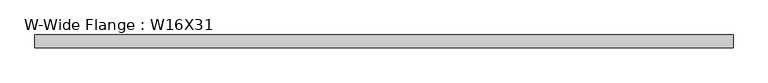
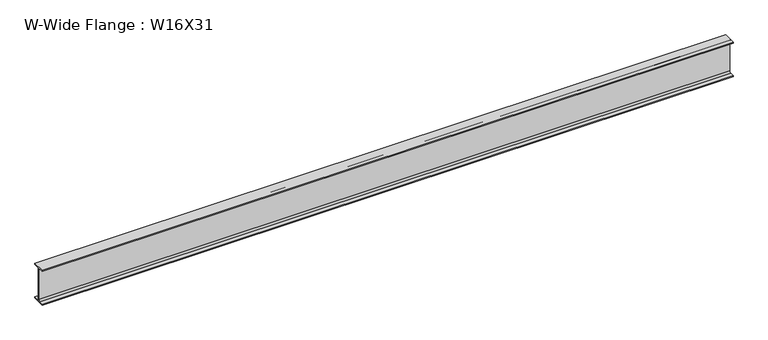
"""IFC4 building model written with IfcOpenShell, lengths in millimetres: beam geometry, W-Wide Flange : W16X31."""

import ifcopenshell
import ifcopenshell.guid

model = None  # the IFC model being written
_history = None  # IfcOwnerHistory: only IFC2X3 demands one
_inside = {}  # id of a spatial element -> (the spatial element, [elements in it])
_under = {}  # id of a project, library or spatial element -> (it, [spatial elements below it])
_declared = {}  # id of a project -> (the project, [libraries it declares])
_typed = {}  # id of a type object -> (the type object, [elements of that type])
_made_of = {}  # id of a material, layer set ... -> (it, [elements and type objects made of it])


def new_model(schema):
    """Start an empty IFC model of exactly this schema.

    Asked for "IFC4X3", IfcOpenShell would pick the latest addendum, in which some entities
    have other attributes; the version numbers below select the first issue.
    IFC2X3 requires an IfcOwnerHistory on every rooted entity: one is made here for all.
    """
    global model, _history
    if schema == "IFC4X3":
        model = ifcopenshell.file(schema_version=(4, 3, 0, 0))
    else:
        model = ifcopenshell.file(schema=schema)
    _inside.clear()
    _under.clear()
    _declared.clear()
    _typed.clear()
    _made_of.clear()
    _history = None
    if model.schema == "IFC2X3":
        org = make("IfcOrganization", Name="unknown")
        user = make(
            "IfcPersonAndOrganization",
            ThePerson=make("IfcPerson", FamilyName="unknown"),
            TheOrganization=org,
        )
        app = make(
            "IfcApplication",
            ApplicationDeveloper=org,
            Version="unknown",
            ApplicationFullName="unknown",
            ApplicationIdentifier="unknown",
        )
        _history = make(
            "IfcOwnerHistory",
            OwningUser=user,
            OwningApplication=app,
            ChangeAction="ADDED",
            CreationDate=0,
        )
    return model


def make(cls, **values):
    """One entity of the class cls with the attributes given. An attribute that is None is left unset."""
    return model.create_entity(
        cls, **{name: value for name, value in values.items() if value is not None}
    )


def rooted(cls, **values):
    """An entity with a GlobalId (a new one), such as an element, a storey or a relation."""
    return make(cls, GlobalId=ifcopenshell.guid.new(), OwnerHistory=_history, **values)


def si_unit(unit_type, name, prefix=None):
    """IfcSIUnit, for example si_unit("LENGTHUNIT", "METRE", prefix="MILLI")."""
    return make("IfcSIUnit", UnitType=unit_type, Prefix=prefix, Name=name)


def assignment(units):
    """IfcUnitAssignment: the units of a project."""
    return None if units is None else make("IfcUnitAssignment", Units=units)


def point(xyz):
    """IfcCartesianPoint."""
    return None if xyz is None else make("IfcCartesianPoint", Coordinates=xyz)


def direction(xyz):
    """IfcDirection."""
    return None if xyz is None else make("IfcDirection", DirectionRatios=xyz)


def frame(location, z_axis=None, x_axis=None):
    """IfcAxis2Placement3D, a coordinate frame: its origin and axes. An axis left out is left unset."""
    return make(
        "IfcAxis2Placement3D",
        Location=point(location),
        Axis=direction(z_axis),
        RefDirection=direction(x_axis),
    )


def frame_2d(location, x_axis=None):
    """IfcAxis2Placement2D, a coordinate frame in the plane: its origin and x axis."""
    return make(
        "IfcAxis2Placement2D", Location=point(location), RefDirection=direction(x_axis)
    )


def origin():
    """The frame at (0, 0, 0) with its axes left unset."""
    return frame((0.0, 0.0, 0.0))


def place(relative_to, where):
    """IfcLocalPlacement: puts the frame where relative to a parent placement (None: the world)."""
    return make(
        "IfcLocalPlacement", PlacementRelTo=relative_to, RelativePlacement=where
    )


def context(
    kind, dimensions, precision=None, world=None, true_north=None, identifier=None
):
    """IfcGeometricRepresentationContext, for example the 3D "Model" context."""
    return make(
        "IfcGeometricRepresentationContext",
        ContextIdentifier=identifier,
        ContextType=kind,
        CoordinateSpaceDimension=dimensions,
        Precision=precision,
        WorldCoordinateSystem=world,
        TrueNorth=true_north,
    )


def project(units=None, contexts=None):
    """IfcProject with its units and contexts."""
    return rooted(
        "IfcProject",
        Name="project",
        RepresentationContexts=contexts,
        UnitsInContext=assignment(units),
    )


def spatial(cls, under=None, at=None, **own):
    """A site, building, storey or space (cls), placed at a placement, below another one or the project."""
    s = rooted(cls, ObjectPlacement=at, **own)
    if under is not None:
        _under.setdefault(under.id(), (under, []))[1].append(s)
    return s


def polyline(points):
    """IfcPolyline through the points."""
    return make("IfcPolyline", Points=[point(p) for p in points])


def circle_curve(where, radius):
    """IfcCircle in the frame where."""
    return make("IfcCircle", Position=where, Radius=radius)


def trimmed(basis, trim1, trim2, sense, master):
    """IfcTrimmedCurve: the piece of a basis curve between two trims."""
    return make(
        "IfcTrimmedCurve",
        BasisCurve=basis,
        Trim1=trim1,
        Trim2=trim2,
        SenseAgreement=sense,
        MasterRepresentation=master,
    )


def segment(curve, same_sense, transition):
    """IfcCompositeCurveSegment."""
    return make(
        "IfcCompositeCurveSegment",
        Transition=transition,
        SameSense=same_sense,
        ParentCurve=curve,
    )


def composite_curve(segments, self_intersect=None):
    """IfcCompositeCurve: segments joined end to end."""
    return make("IfcCompositeCurve", Segments=segments, SelfIntersect=self_intersect)


def outline(outer, holes=None, kind="AREA"):
    """IfcArbitraryClosedProfileDef: a profile drawn as a closed curve; with holes, ...WithVoids."""
    if holes is None:
        return make("IfcArbitraryClosedProfileDef", ProfileType=kind, OuterCurve=outer)
    return make(
        "IfcArbitraryProfileDefWithVoids",
        ProfileType=kind,
        OuterCurve=outer,
        InnerCurves=holes,
    )


def extrude(swept, where, along, depth):
    """IfcExtrudedAreaSolid: the profile swept, set in the frame where, extruded along a direction by depth."""
    return make(
        "IfcExtrudedAreaSolid",
        SweptArea=swept,
        Position=where,
        ExtrudedDirection=direction(along),
        Depth=depth,
    )


def shape(context_of_items, identifier, shape_type, items):
    """IfcShapeRepresentation: the items that make up one representation, for example the "Body"."""
    return make(
        "IfcShapeRepresentation",
        ContextOfItems=context_of_items,
        RepresentationIdentifier=identifier,
        RepresentationType=shape_type,
        Items=items,
    )


def source(mapping_origin, context_of_items, identifier, shape_type, items):
    """IfcRepresentationMap: a shape defined once, which mapped items show again and again."""
    return make(
        "IfcRepresentationMap",
        MappingOrigin=mapping_origin,
        MappedRepresentation=shape(context_of_items, identifier, shape_type, items),
    )


def transform(
    local_origin,
    x_axis=None,
    y_axis=None,
    z_axis=None,
    scale=None,
    scale2=None,
    scale3=None,
    uniform=True,
):
    """IfcCartesianTransformationOperator3D, or its non-uniform kind. x_axis, y_axis, z_axis: its Axis1, 2, 3."""
    if uniform:
        return make(
            "IfcCartesianTransformationOperator3D",
            Axis1=direction(x_axis),
            Axis2=direction(y_axis),
            LocalOrigin=point(local_origin),
            Scale=scale,
            Axis3=direction(z_axis),
        )
    return make(
        "IfcCartesianTransformationOperator3DnonUniform",
        Axis1=direction(x_axis),
        Axis2=direction(y_axis),
        LocalOrigin=point(local_origin),
        Scale=scale,
        Axis3=direction(z_axis),
        Scale2=scale2,
        Scale3=scale3,
    )


def mapped(mapping_source, mapping_target):
    """IfcMappedItem: shows the shape of a source again, moved by a transform."""
    return make(
        "IfcMappedItem", MappingSource=mapping_source, MappingTarget=mapping_target
    )


def made_of(thing, what):
    """Note that an element or type object is made of a material, layer set ...; save() writes the relation."""
    if what is not None:
        _made_of.setdefault(what.id(), (what, []))[1].append(thing)
    return thing


def element(
    cls,
    number,
    at=None,
    inside=None,
    cuts=None,
    type_object=None,
    material=None,
    context=None,
    identifier="Body",
    shape_type=None,
    held_by="IfcProductDefinitionShape",
    body=None,
    shapes=None,
    **own,
):
    """One element of the class cls, such as IfcWall. Its Tag is "e" and its number.

    at: its placement. inside: the storey or other place that contains it. cuts: it is an
    opening in that element (IfcRelVoidsElement). A single representation is given by context,
    identifier, shape_type and body (its items); several are given by shapes. held_by: the class
    of the entity that holds the representations. save() writes the other relations.
    """
    e = rooted(cls, Tag="e%d" % number, ObjectPlacement=at, **own)
    if body is not None:
        shapes = [shape(context, identifier, shape_type, body)]
    if shapes is not None:
        e.Representation = make(held_by, Representations=shapes)
    if inside is not None:
        _inside.setdefault(inside.id(), (inside, []))[1].append(e)
    if cuts is not None:
        rooted(
            "IfcRelVoidsElement", RelatingBuildingElement=cuts, RelatedOpeningElement=e
        )
    if type_object is not None:
        _typed.setdefault(type_object.id(), (type_object, []))[1].append(e)
    return made_of(e, material)


def aggregate(whole, parts):
    """IfcRelAggregates: a whole, such as a stair, and the parts it consists of."""
    return rooted("IfcRelAggregates", RelatingObject=whole, RelatedObjects=parts)


def save(model, path):
    """Write the relations noted so far, then the file.

    IfcRelAggregates (storeys below a building ...), IfcRelContainedInSpatialStructure (elements
    in a storey), IfcRelDefinesByType, IfcRelAssociatesMaterial and IfcRelDeclares: one each for
    every whole, place, type object, material and project.
    """
    for whole, parts in _under.values():
        aggregate(whole, parts)
    for where, things in _inside.values():
        rooted(
            "IfcRelContainedInSpatialStructure",
            RelatedElements=things,
            RelatingStructure=where,
        )
    for kind, things in _typed.values():
        rooted("IfcRelDefinesByType", RelatedObjects=things, RelatingType=kind)
    for what, things in _made_of.values():
        rooted("IfcRelAssociatesMaterial", RelatedObjects=things, RelatingMaterial=what)
    for by, libraries in _declared.values():
        rooted("IfcRelDeclares", RelatingContext=by, RelatedDefinitions=libraries)
    model.write(path)


def w_wide_flange_w16x31_348d06aa(model_context):
    return source(origin(), model_context, "Body", "SweptSolid", [
        extrude(outline(composite_curve([segment(polyline([(70.231, -190.754), (70.231, -201.93), (-70.231, -201.93), (-70.231, -190.754), (-20.8915, -190.754)]), True, "CONTINUOUS"), segment(trimmed(circle_curve(frame_2d((-20.8915, -173.355)), 17.399), [point((-20.8915, -190.754))], [point((-3.4925, -173.355))], True, "CARTESIAN"), True, "CONTINUOUS"), segment(polyline([(-3.4925, -173.355), (-3.4925, 173.355)]), True, "CONTINUOUS"), segment(trimmed(circle_curve(frame_2d((-20.8915, 173.355)), 17.399), [point((-3.4925, 173.355))], [point((-20.8915, 190.754))], True, "CARTESIAN"), True, "CONTINUOUS"), segment(polyline([(-20.8915, 190.754), (-70.231, 190.754), (-70.231, 201.93), (70.231, 201.93), (70.231, 190.754), (20.8915, 190.754)]), True, "CONTINUOUS"), segment(trimmed(circle_curve(frame_2d((20.8915, 173.355)), 17.399), [point((20.8915, 190.754))], [point((3.4925, 173.355))], True, "CARTESIAN"), True, "CONTINUOUS"), segment(polyline([(3.4925, 173.355), (3.4925, -173.355)]), True, "CONTINUOUS"), segment(trimmed(circle_curve(frame_2d((20.8915, -173.355)), 17.399), [point((3.4925, -173.355))], [point((20.8915, -190.754))], True, "CARTESIAN"), True, "CONTINUOUS"), segment(polyline([(20.8915, -190.754), (70.231, -190.754)]), True, "CONTINUOUS")], self_intersect=False)), frame((-3784.6209019, 0.0, 0.0), z_axis=(1.0, 0.0, 0.0), x_axis=(0.0, 1.0, 0.0)), (0.0, 0.0, 1.0), 7625.969),
    ])


if __name__ == "__main__":
    model = new_model("IFC4")
    model_context = context("Model", 3, world=origin())
    ifc_project = project(units=[si_unit("LENGTHUNIT", "METRE", prefix="MILLI")], contexts=[model_context])
    site = spatial("IfcSite", under=ifc_project)
    building = spatial("IfcBuilding", under=site)
    placement = place(None, origin())
    w_wide_flange_w16x31_shape = w_wide_flange_w16x31_348d06aa(model_context)
    element("IfcBeam", 1, ObjectType="W-Wide Flange : W16X31", at=placement, inside=building, context=model_context, shape_type="MappedRepresentation", body=[
        mapped(w_wide_flange_w16x31_shape, transform((0.0, 0.0, 0.0), x_axis=(1.0, 0.0, 0.0), y_axis=(0.0, 1.0, 0.0), z_axis=(0.0, 0.0, 1.0))),
    ])
    save(model, "model.ifc")

# Revit data of these elements
# Type "W-Wide Flange : W16X31"
#   Assembly Code = "B10"
#   W = 31
#   Start Extension Calculation [instance default] = 10' - 0"
#   Start Extension [instance default] = -0' - 0 1/2"
#   End Extension Calculation [instance default] = 10' - 0"
#   End Extension [instance default] = -0' - 0 1/2"
#   Length [instance default] = 5' - 0"
#   bf = 0' - 5.53"
#   d = 1' - 3.9"
#   k = 0' - 1 1/8"
#   k2 = 0' - 0.685"
#   tf = 0' - 0.44"
#   tw = 0' - 0.275"
#   A = 0.0634028 SF
#   Beam Material [instance default] = Metal - Steel - ASTM A992
# Element 1 (IfcBeam, "W-Wide Flange : W16X31")
#   Materials on its faces: "Metal - Steel - ASTM A992"
# Materials
#   "Metal - Steel - ASTM A992": class "Metal", colour RGB 128 0 0, transparency 0
